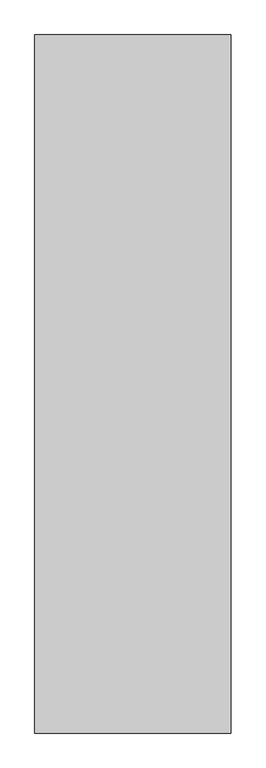
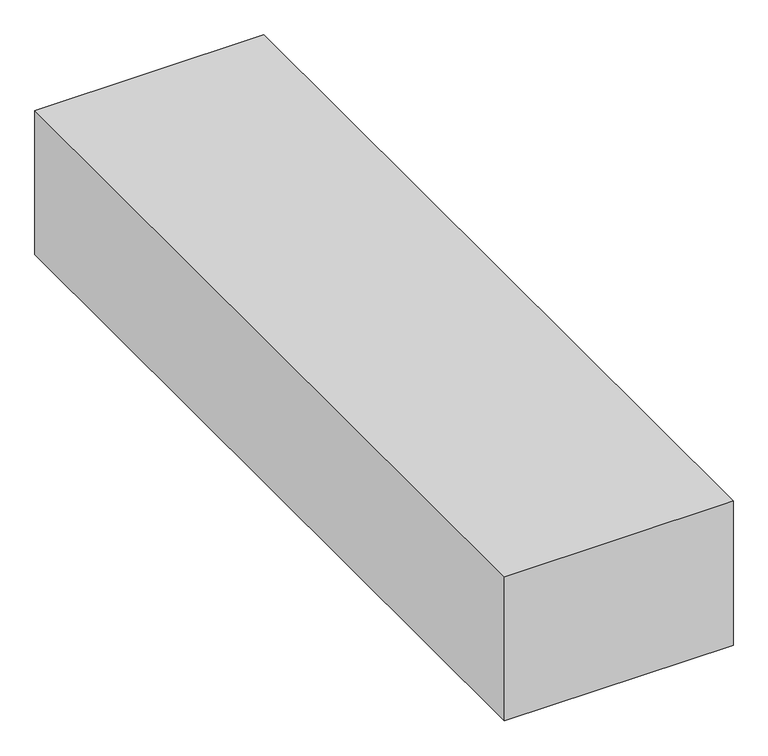
"""IFC4 building model written with IfcOpenShell, lengths in millimetres: proxy geometry, Space Planning Box_hec : Space Planning Box_hec."""

from ifc_helpers import new_model, si_unit, origin, origin_with_axes, place, context, project, spatial, polyline, outline, extrude, source, transform, mapped, element, save


def generic_models_57c7875f(model_context):
    return source(origin(), model_context, "Body", "SweptSolid", [
        extrude(outline(polyline([(4500.0, 16000.0), (4500.0, -16000.0), (-4500.0, -16000.0), (-4500.0, 16000.0), (4500.0, 16000.0)])), origin_with_axes(), (0.0, 0.0, 1.0), 6000.0),
    ])


if __name__ == "__main__":
    model = new_model("IFC4")
    model_context = context("Model", 3, world=origin())
    ifc_project = project(units=[si_unit("LENGTHUNIT", "METRE", prefix="MILLI")], contexts=[model_context])
    site = spatial("IfcSite", under=ifc_project)
    building = spatial("IfcBuilding", under=site)
    placement = place(None, origin())
    generic_models_shape = generic_models_57c7875f(model_context)
    element("IfcBuildingElementProxy", 1, Name="Space Planning Box_hec : Space Planning Box_hec", ObjectType="Space Planning Box_hec : Space Planning Box_hec", at=placement, inside=building, context=model_context, shape_type="MappedRepresentation", body=[
        mapped(generic_models_shape, transform((0.0, 0.0, 0.0), x_axis=(1.0, 0.0, 0.0), y_axis=(0.0, 1.0, 0.0), z_axis=(0.0, 0.0, 1.0))),
    ])
    save(model, "model.ifc")

# Revit data of these elements
# Type "Space Planning Box_hec : Space Planning Box_hec"
#   Type Comments = "..."
#   Room Name [instance default] = "?"
#   Interior Finish [instance default] = ""
#   Exterior Finish [instance default] = ""
#   Department [instance default] = ""
#   Assembly Code = "..."
#   Width [instance default] = 1524 mm
#   Program Area [instance default] = 0 m²
#   Length [instance default] = 1524 mm
#   Height [instance default] = 1524 mm
#   Area [instance default] = 2.32258 m²
#   Fill Color [instance default] = Cyan
#   Default Elevation = 0
# Element 1 (IfcBuildingElementProxy, "Space Planning Box_hec : Space Planning Box_hec")
#   Room Name = "Central Control Room"
#   Interior Finish = "IF3"
#   Exterior Finish = "EF1"
#   Department = "CI"
#   Width = 9000 mm
#   Program Area = 288 m²
#   Length = 32000 mm
#   Height = 6000 mm
#   Area = 288 m²
#   Fill Color = Lime
#   Materials on its faces: "Lime"
# Materials
#   "Cyan": class "Generic", colour RGB 0 255 255, transparency 0.2, Cost = 0
#   "Lime": class "Generic", colour RGB 0 255 0, transparency 0.2, Cost = 0
